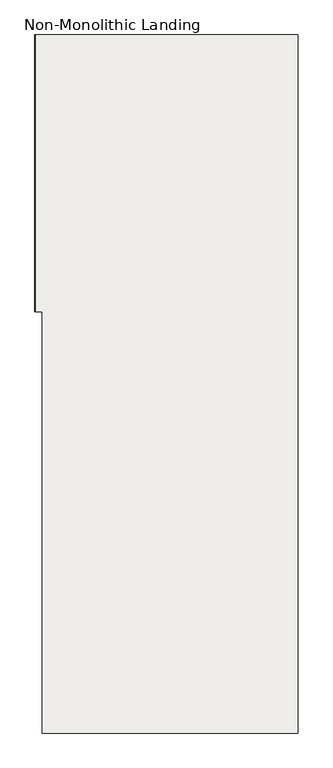
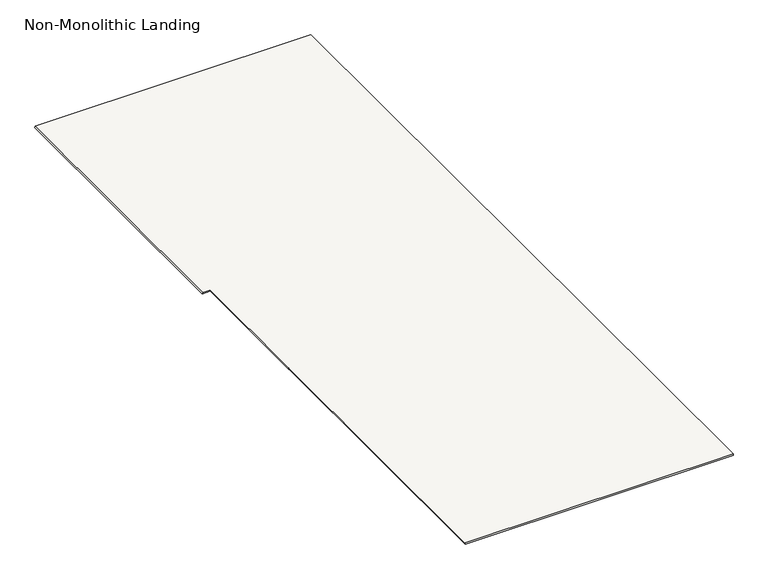
"""IFC4 building model written with IfcOpenShell, lengths in millimetres: slab geometry, Non-Monolithic Landing."""

from ifc_helpers import new_model, si_unit, origin, place, context, project, spatial, faceted_brep, source, transform, mapped, element, save


def non_monolithic_landing_65127f9e(model_context):
    return source(origin(), model_context, "Body", "Brep", [
        faceted_brep([(16318.9400908, 13220.4345331, 18411.7647059), (16318.0900908, 13220.4345331, 18405.7647059), (16318.0900908, 12030.4345331, 18405.7647059), (16318.9400908, 12030.4345331, 18411.7647059), (16350.0, 10220.4345331, 18411.7647059), (17450.0, 10220.4345331, 18411.7647059), (17450.0, 13220.4345331, 18411.7647059), (16350.0, 13220.4345331, 18411.7647059), (16350.0, 12030.4345331, 18411.7647059), (16350.0, 11470.4345331, 18411.7647059), (17450.0, 13220.4345331, 18405.7647059), (17450.0, 10220.4345331, 18405.7647059), (16350.85, 10220.4345331, 18405.7647059), (16350.85, 11470.4345331, 18405.7647059), (16350.0, 11470.4345331, 18405.7647059), (16350.0, 12030.4345331, 18405.7647059), (16350.0, 13220.4345331, 18405.7647059)], [[[0, 1, 2, 3]], [[4, 5, 6, 7, 0, 3, 8, 9]], [[10, 11, 12, 13, 14, 15, 2, 1, 16]], [[9, 8, 15, 14]], [[0, 7, 16, 1]], [[7, 6, 10, 16]], [[6, 5, 11, 10]], [[5, 4, 12, 11]], [[13, 9, 14]], [[9, 13, 12, 4]], [[8, 3, 2, 15]]]),
    ])


if __name__ == "__main__":
    model = new_model("IFC4")
    model_context = context("Model", 3, world=origin())
    ifc_project = project(units=[si_unit("LENGTHUNIT", "METRE", prefix="MILLI")], contexts=[model_context])
    site = spatial("IfcSite", under=ifc_project)
    building = spatial("IfcBuilding", under=site)
    placement = place(None, origin())
    non_monolithic_landing_shape = non_monolithic_landing_65127f9e(model_context)
    element("IfcSlab", 1, ObjectType="Non-Monolithic Landing", at=placement, inside=building, context=model_context, shape_type="MappedRepresentation", body=[
        mapped(non_monolithic_landing_shape, transform((0.0, 0.0, 0.0), x_axis=(1.0, 0.0, 0.0), y_axis=(0.0, 1.0, 0.0), z_axis=(0.0, 0.0, 1.0))),
    ])
    save(model, "model.ifc")

# Revit data of these elements
# Element 1 (IfcSlab, "Non-Monolithic Landing")
#   Materials on its faces: "Steel, Paint Finish, Dark Gray"
# Materials
#   "Steel, Paint Finish, Dark Gray": class "Metal", colour RGB 89 89 89, transparency 0, Description = "Steel, paint finish, dark gray, glossy", Cost = 0
